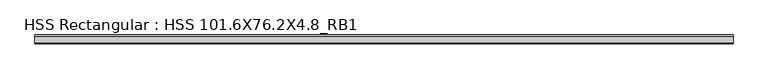
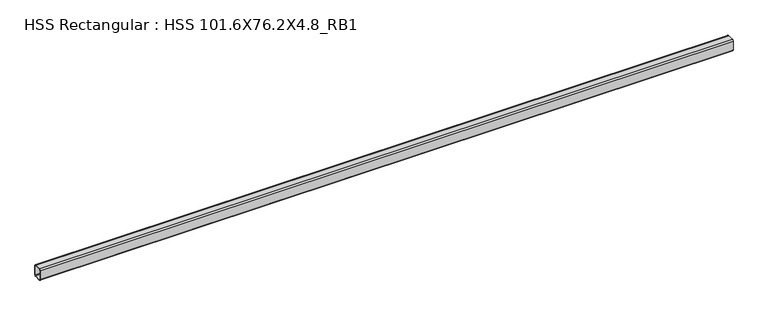
"""IFC4 building model written with IfcOpenShell, lengths in millimetres: beam geometry, HSS Rectangular : HSS 101.6X76.2X4.8_RB1."""

from ifc_helpers import new_model, si_unit, point, frame, frame_2d, origin, place, context, project, spatial, polyline, circle_curve, trimmed, segment, composite_curve, outline, extrude, source, transform, mapped, element, save


def hss_rectangular_hss_101_6x76_2x4_8_rb1_2e336e92(model_context):
    return source(origin(), model_context, "Body", "SweptSolid", [
        extrude(outline(composite_curve([segment(polyline([(38.1, 41.275), (38.1, -41.275)]), True, "CONTINUOUS"), segment(trimmed(circle_curve(frame_2d((28.575, -41.275)), 9.525), [point((38.1, -41.275))], [point((28.575, -50.8))], False, "CARTESIAN"), True, "CONTINUOUS"), segment(polyline([(28.575, -50.8), (-28.575, -50.8)]), True, "CONTINUOUS"), segment(trimmed(circle_curve(frame_2d((-28.575, -41.275)), 9.525), [point((-28.575, -50.8))], [point((-38.1, -41.275))], False, "CARTESIAN"), True, "CONTINUOUS"), segment(polyline([(-38.1, -41.275), (-38.1, 41.275)]), True, "CONTINUOUS"), segment(trimmed(circle_curve(frame_2d((-28.575, 41.275)), 9.525), [point((-38.1, 41.275))], [point((-28.575, 50.8))], False, "CARTESIAN"), True, "CONTINUOUS"), segment(polyline([(-28.575, 50.8), (28.575, 50.8)]), True, "CONTINUOUS"), segment(trimmed(circle_curve(frame_2d((28.575, 41.275)), 9.525), [point((28.575, 50.8))], [point((38.1, 41.275))], False, "CARTESIAN"), True, "CONTINUOUS")], self_intersect=False), holes=[composite_curve([segment(trimmed(circle_curve(frame_2d((-28.575, 41.275)), 4.7625), [point((-28.575, 46.0375))], [point((-33.3375, 41.275))], True, "CARTESIAN"), True, "CONTINUOUS"), segment(polyline([(-33.3375, 41.275), (-33.3375, -41.275)]), True, "CONTINUOUS"), segment(trimmed(circle_curve(frame_2d((-28.575, -41.275)), 4.7625), [point((-33.3375, -41.275))], [point((-28.575, -46.0375))], True, "CARTESIAN"), True, "CONTINUOUS"), segment(polyline([(-28.575, -46.0375), (28.575, -46.0375)]), True, "CONTINUOUS"), segment(trimmed(circle_curve(frame_2d((28.575, -41.275)), 4.7625), [point((28.575, -46.0375))], [point((33.3375, -41.275))], True, "CARTESIAN"), True, "CONTINUOUS"), segment(polyline([(33.3375, -41.275), (33.3375, 41.275)]), True, "CONTINUOUS"), segment(trimmed(circle_curve(frame_2d((28.575, 41.275)), 4.7625), [point((33.3375, 41.275))], [point((28.575, 46.0375))], True, "CARTESIAN"), True, "CONTINUOUS"), segment(polyline([(28.575, 46.0375), (-28.575, 46.0375)]), True, "CONTINUOUS")], self_intersect=False)]), frame((-7493.3247032, 0.0, 0.0), z_axis=(1.0, 0.0, 0.0), x_axis=(0.0, 1.0, 0.0)), (0.0, 0.0, 1.0), 5965.3362894),
    ])


if __name__ == "__main__":
    model = new_model("IFC4")
    model_context = context("Model", 3, world=origin())
    ifc_project = project(units=[si_unit("LENGTHUNIT", "METRE", prefix="MILLI")], contexts=[model_context])
    site = spatial("IfcSite", under=ifc_project)
    building = spatial("IfcBuilding", under=site)
    placement = place(None, origin())
    hss_rectangular_hss_101_6x76_2x4_8_rb1_shape = hss_rectangular_hss_101_6x76_2x4_8_rb1_2e336e92(model_context)
    element("IfcBeam", 1, ObjectType="HSS Rectangular : HSS 101.6X76.2X4.8_RB1", at=placement, inside=building, context=model_context, shape_type="MappedRepresentation", body=[
        mapped(hss_rectangular_hss_101_6x76_2x4_8_rb1_shape, transform((0.0, 0.0, 0.0), x_axis=(1.0, 0.0, 0.0), y_axis=(0.0, 1.0, 0.0), z_axis=(0.0, 0.0, 1.0))),
    ])
    save(model, "model.ifc")

# Revit data of these elements
# Type "HSS Rectangular : HSS 101.6X76.2X4.8_RB1"
#   Section Name Key = "HSS 4X3X3/16"
#   Assembly Code = "B10"
#   Width = 7.62 cm
#   Wall Nominal Thickness = 0.4763 cm
#   Wall Design Thickness = 0.442 cm
#   Torsional Moment of Inertia = 260.561 cm⁴
#   Torsional Modulus = 61.2876 cm³
#   Section Area = 14.4516 cm²
#   Plastic Modulus weak axis = 40.3122 cm³
#   Plastic Modulus strong axis = 49.1612 cm³
#   Perimeter = 0.881482 m²/m
#   Outer Fillet = 0.9525 cm
#   Nominal Weight = 12.1285 kgf/m
#   Moment of Inertia weak axis = 131.529 cm⁴
#   Moment of Inertia strong axis = 205.202 cm⁴
#   Inner Fillet = 0.4763 cm
#   Height = 10.16 cm
#   Elastic Modulus weak axis = 34.4128 cm³
#   Elastic Modulus strong axis = 40.476 cm³
#   Centroid Vertical = 5.08 cm
#   Centroid Horizontal = 3.81 cm
#   Length [instance default] = 1524 mm
#   Structural Material [instance default] = Steel ASTM A500, Grade B, Rectangular and Square
#   Principal Axes Angle = 0
# Element 1 (IfcBeam, "HSS Rectangular : HSS 101.6X76.2X4.8_RB1")
#   Structural Material = Steel ASTM A992
#   Materials on its faces: "Steel ASTM A992"
# Materials
#   "Steel ASTM A500, Grade B, Rectangular and Square": class "Metal", colour RGB 199 199 199, transparency 0, Description = "Carbon steel", Cost = 0
#   "Steel ASTM A992": class "Metal", colour RGB 199 199 199, transparency 0, Description = "Structural steel 50ksi", Cost = 0
